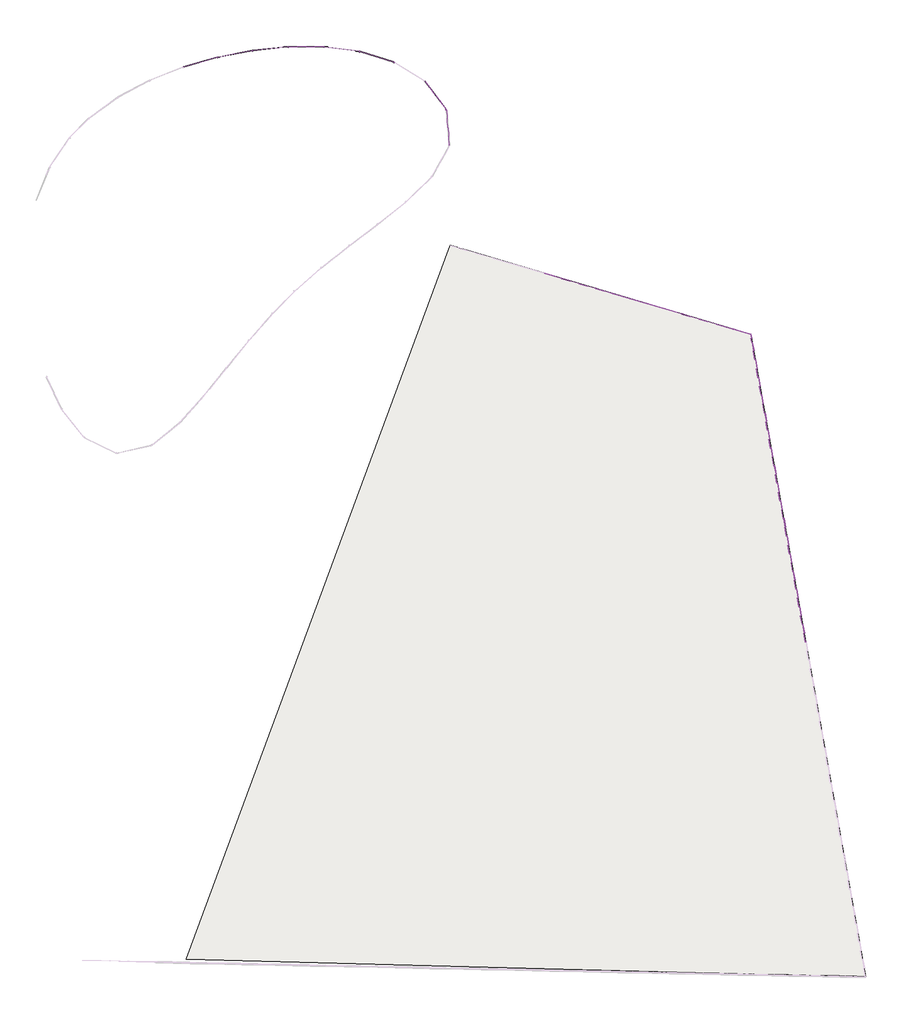
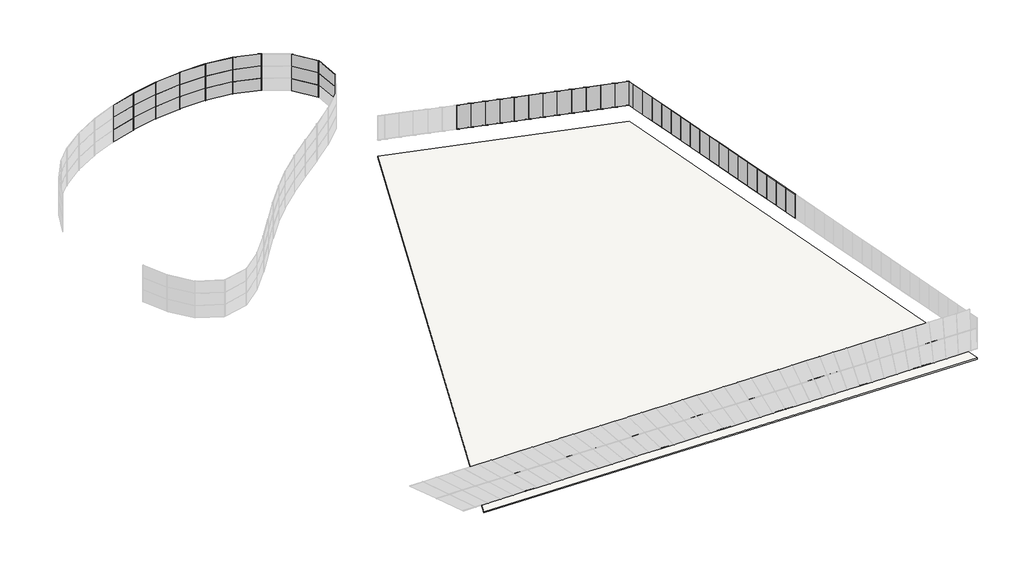
# One storey, part 5 of 5: 53 plates, 51 members, 1 slab.
"""IFC4 building model written with IfcOpenShell, lengths in millimetres."""

import ifcopenshell
import ifcopenshell.guid

model = None  # the IFC model being written
_history = None  # IfcOwnerHistory: only IFC2X3 demands one
_inside = {}  # id of a spatial element -> (the spatial element, [elements in it])
_under = {}  # id of a project, library or spatial element -> (it, [spatial elements below it])
_declared = {}  # id of a project -> (the project, [libraries it declares])
_typed = {}  # id of a type object -> (the type object, [elements of that type])
_made_of = {}  # id of a material, layer set ... -> (it, [elements and type objects made of it])


def new_model(schema):
    """Start an empty IFC model of exactly this schema.

    Asked for "IFC4X3", IfcOpenShell would pick the latest addendum, in which some entities
    have other attributes; the version numbers below select the first issue.
    IFC2X3 requires an IfcOwnerHistory on every rooted entity: one is made here for all.
    """
    global model, _history
    if schema == "IFC4X3":
        model = ifcopenshell.file(schema_version=(4, 3, 0, 0))
    else:
        model = ifcopenshell.file(schema=schema)
    _inside.clear()
    _under.clear()
    _declared.clear()
    _typed.clear()
    _made_of.clear()
    _history = None
    if model.schema == "IFC2X3":
        org = make("IfcOrganization", Name="unknown")
        user = make(
            "IfcPersonAndOrganization",
            ThePerson=make("IfcPerson", FamilyName="unknown"),
            TheOrganization=org,
        )
        app = make(
            "IfcApplication",
            ApplicationDeveloper=org,
            Version="unknown",
            ApplicationFullName="unknown",
            ApplicationIdentifier="unknown",
        )
        _history = make(
            "IfcOwnerHistory",
            OwningUser=user,
            OwningApplication=app,
            ChangeAction="ADDED",
            CreationDate=0,
        )
    return model


def make(cls, **values):
    """One entity of the class cls with the attributes given. An attribute that is None is left unset."""
    return model.create_entity(
        cls, **{name: value for name, value in values.items() if value is not None}
    )


def rooted(cls, **values):
    """An entity with a GlobalId (a new one), such as an element, a storey or a relation."""
    return make(cls, GlobalId=ifcopenshell.guid.new(), OwnerHistory=_history, **values)


def si_unit(unit_type, name, prefix=None):
    """IfcSIUnit, for example si_unit("LENGTHUNIT", "METRE", prefix="MILLI")."""
    return make("IfcSIUnit", UnitType=unit_type, Prefix=prefix, Name=name)


def assignment(units):
    """IfcUnitAssignment: the units of a project."""
    return None if units is None else make("IfcUnitAssignment", Units=units)


def point(xyz):
    """IfcCartesianPoint."""
    return None if xyz is None else make("IfcCartesianPoint", Coordinates=xyz)


def direction(xyz):
    """IfcDirection."""
    return None if xyz is None else make("IfcDirection", DirectionRatios=xyz)


def frame(location, z_axis=None, x_axis=None):
    """IfcAxis2Placement3D, a coordinate frame: its origin and axes. An axis left out is left unset."""
    return make(
        "IfcAxis2Placement3D",
        Location=point(location),
        Axis=direction(z_axis),
        RefDirection=direction(x_axis),
    )


def frame_2d(location, x_axis=None):
    """IfcAxis2Placement2D, a coordinate frame in the plane: its origin and x axis."""
    return make(
        "IfcAxis2Placement2D", Location=point(location), RefDirection=direction(x_axis)
    )


def origin():
    """The frame at (0, 0, 0) with its axes left unset."""
    return frame((0.0, 0.0, 0.0))


def origin_with_axes():
    """The frame at (0, 0, 0) with the z axis (0, 0, 1) and the x axis (1, 0, 0) written out."""
    return frame((0.0, 0.0, 0.0), z_axis=(0.0, 0.0, 1.0), x_axis=(1.0, 0.0, 0.0))


def origin_2d():
    """The frame at (0, 0) in the plane with its x axis left unset."""
    return frame_2d((0.0, 0.0))


def place(relative_to, where):
    """IfcLocalPlacement: puts the frame where relative to a parent placement (None: the world)."""
    return make(
        "IfcLocalPlacement", PlacementRelTo=relative_to, RelativePlacement=where
    )


def context(
    kind, dimensions, precision=None, world=None, true_north=None, identifier=None
):
    """IfcGeometricRepresentationContext, for example the 3D "Model" context."""
    return make(
        "IfcGeometricRepresentationContext",
        ContextIdentifier=identifier,
        ContextType=kind,
        CoordinateSpaceDimension=dimensions,
        Precision=precision,
        WorldCoordinateSystem=world,
        TrueNorth=true_north,
    )


def project(units=None, contexts=None):
    """IfcProject with its units and contexts."""
    return rooted(
        "IfcProject",
        Name="project",
        RepresentationContexts=contexts,
        UnitsInContext=assignment(units),
    )


def spatial(cls, under=None, at=None, **own):
    """A site, building, storey or space (cls), placed at a placement, below another one or the project."""
    s = rooted(cls, ObjectPlacement=at, **own)
    if under is not None:
        _under.setdefault(under.id(), (under, []))[1].append(s)
    return s


def polyline(points):
    """IfcPolyline through the points."""
    return make("IfcPolyline", Points=[point(p) for p in points])


def circle_curve(where, radius):
    """IfcCircle in the frame where."""
    return make("IfcCircle", Position=where, Radius=radius)


def trimmed(basis, trim1, trim2, sense, master):
    """IfcTrimmedCurve: the piece of a basis curve between two trims."""
    return make(
        "IfcTrimmedCurve",
        BasisCurve=basis,
        Trim1=trim1,
        Trim2=trim2,
        SenseAgreement=sense,
        MasterRepresentation=master,
    )


def segment(curve, same_sense, transition):
    """IfcCompositeCurveSegment."""
    return make(
        "IfcCompositeCurveSegment",
        Transition=transition,
        SameSense=same_sense,
        ParentCurve=curve,
    )


def composite_curve(segments, self_intersect=None):
    """IfcCompositeCurve: segments joined end to end."""
    return make("IfcCompositeCurve", Segments=segments, SelfIntersect=self_intersect)


def outline(outer, holes=None, kind="AREA"):
    """IfcArbitraryClosedProfileDef: a profile drawn as a closed curve; with holes, ...WithVoids."""
    if holes is None:
        return make("IfcArbitraryClosedProfileDef", ProfileType=kind, OuterCurve=outer)
    return make(
        "IfcArbitraryProfileDefWithVoids",
        ProfileType=kind,
        OuterCurve=outer,
        InnerCurves=holes,
    )


def extrude(swept, where, along, depth):
    """IfcExtrudedAreaSolid: the profile swept, set in the frame where, extruded along a direction by depth."""
    return make(
        "IfcExtrudedAreaSolid",
        SweptArea=swept,
        Position=where,
        ExtrudedDirection=direction(along),
        Depth=depth,
    )


def shape(context_of_items, identifier, shape_type, items):
    """IfcShapeRepresentation: the items that make up one representation, for example the "Body"."""
    return make(
        "IfcShapeRepresentation",
        ContextOfItems=context_of_items,
        RepresentationIdentifier=identifier,
        RepresentationType=shape_type,
        Items=items,
    )


def source(mapping_origin, context_of_items, identifier, shape_type, items):
    """IfcRepresentationMap: a shape defined once, which mapped items show again and again."""
    return make(
        "IfcRepresentationMap",
        MappingOrigin=mapping_origin,
        MappedRepresentation=shape(context_of_items, identifier, shape_type, items),
    )


def transform(
    local_origin,
    x_axis=None,
    y_axis=None,
    z_axis=None,
    scale=None,
    scale2=None,
    scale3=None,
    uniform=True,
):
    """IfcCartesianTransformationOperator3D, or its non-uniform kind. x_axis, y_axis, z_axis: its Axis1, 2, 3."""
    if uniform:
        return make(
            "IfcCartesianTransformationOperator3D",
            Axis1=direction(x_axis),
            Axis2=direction(y_axis),
            LocalOrigin=point(local_origin),
            Scale=scale,
            Axis3=direction(z_axis),
        )
    return make(
        "IfcCartesianTransformationOperator3DnonUniform",
        Axis1=direction(x_axis),
        Axis2=direction(y_axis),
        LocalOrigin=point(local_origin),
        Scale=scale,
        Axis3=direction(z_axis),
        Scale2=scale2,
        Scale3=scale3,
    )


def mapped(mapping_source, mapping_target):
    """IfcMappedItem: shows the shape of a source again, moved by a transform."""
    return make(
        "IfcMappedItem", MappingSource=mapping_source, MappingTarget=mapping_target
    )


def made_of(thing, what):
    """Note that an element or type object is made of a material, layer set ...; save() writes the relation."""
    if what is not None:
        _made_of.setdefault(what.id(), (what, []))[1].append(thing)
    return thing


def element(
    cls,
    number,
    at=None,
    inside=None,
    cuts=None,
    type_object=None,
    material=None,
    context=None,
    identifier="Body",
    shape_type=None,
    held_by="IfcProductDefinitionShape",
    body=None,
    shapes=None,
    **own,
):
    """One element of the class cls, such as IfcWall. Its Tag is "e" and its number.

    at: its placement. inside: the storey or other place that contains it. cuts: it is an
    opening in that element (IfcRelVoidsElement). A single representation is given by context,
    identifier, shape_type and body (its items); several are given by shapes. held_by: the class
    of the entity that holds the representations. save() writes the other relations.
    """
    e = rooted(cls, Tag="e%d" % number, ObjectPlacement=at, **own)
    if body is not None:
        shapes = [shape(context, identifier, shape_type, body)]
    if shapes is not None:
        e.Representation = make(held_by, Representations=shapes)
    if inside is not None:
        _inside.setdefault(inside.id(), (inside, []))[1].append(e)
    if cuts is not None:
        rooted(
            "IfcRelVoidsElement", RelatingBuildingElement=cuts, RelatedOpeningElement=e
        )
    if type_object is not None:
        _typed.setdefault(type_object.id(), (type_object, []))[1].append(e)
    return made_of(e, material)


def aggregate(whole, parts):
    """IfcRelAggregates: a whole, such as a stair, and the parts it consists of."""
    return rooted("IfcRelAggregates", RelatingObject=whole, RelatedObjects=parts)


def save(model, path):
    """Write the relations noted so far, then the file.

    IfcRelAggregates (storeys below a building ...), IfcRelContainedInSpatialStructure (elements
    in a storey), IfcRelDefinesByType, IfcRelAssociatesMaterial and IfcRelDeclares: one each for
    every whole, place, type object, material and project.
    """
    for whole, parts in _under.values():
        aggregate(whole, parts)
    for where, things in _inside.values():
        rooted(
            "IfcRelContainedInSpatialStructure",
            RelatedElements=things,
            RelatingStructure=where,
        )
    for kind, things in _typed.values():
        rooted("IfcRelDefinesByType", RelatedObjects=things, RelatingType=kind)
    for what, things in _made_of.values():
        rooted("IfcRelAssociatesMaterial", RelatedObjects=things, RelatingMaterial=what)
    for by, libraries in _declared.values():
        rooted("IfcRelDeclares", RelatingContext=by, RelatedDefinitions=libraries)
    model.write(path)


def montante_circular_25_mm_raio_36e581cf(model_context):
    return source(origin(), model_context, "Body", "SweptSolid", [
        extrude(outline(composite_curve([segment(trimmed(circle_curve(origin_2d(), 25.0), [point((25.0, 0.0))], [point((-25.0, 0.0))], False, "CARTESIAN"), True, "CONTINUOUS"), segment(trimmed(circle_curve(origin_2d(), 25.0), [point((-25.0, 0.0))], [point((25.0, 0.0))], False, "CARTESIAN"), True, "CONTINUOUS")], self_intersect=False)), frame((0.0, 0.0, -1500.0), z_axis=(0.0, 0.0, 1.0), x_axis=(1.0, 0.0, 0.0)), (0.0, 0.0, 1.0), 1500.0),
    ])


def montante_circular_25_mm_raio_b6a72e74(model_context):
    return source(origin(), model_context, "Body", "SweptSolid", [
        extrude(outline(composite_curve([segment(trimmed(circle_curve(origin_2d(), 25.0), [point((25.0, 0.0))], [point((-25.0, 0.0))], False, "CARTESIAN"), True, "CONTINUOUS"), segment(trimmed(circle_curve(origin_2d(), 25.0), [point((-25.0, 0.0))], [point((25.0, 0.0))], False, "CARTESIAN"), True, "CONTINUOUS")], self_intersect=False)), frame((0.0, 0.0, -685.7133319), z_axis=(0.0, 0.0, 1.0), x_axis=(1.0, 0.0, 0.0)), (0.0, 0.0, 1.0), 685.7133319),
    ])


def painel_do_sistema_5ef9eced(model_context):
    return source(origin(), model_context, "Body", "SweptSolid", [
        extrude(outline(polyline([(1475.0, 24.5), (-1475.0, 24.5), (-1475.0, 49.5), (1475.0, 49.5), (1475.0, 24.5)])), origin_with_axes(), (0.0, 0.0, 1.0), 1500.0),
    ])


def painel_do_sistema_14e00207(model_context):
    return source(origin(), model_context, "Body", "SweptSolid", [
        extrude(outline(polyline([(1475.0, 24.5), (-1475.0, 24.5), (-1475.0, 49.5), (1475.0, 49.5), (1475.0, 24.5)])), origin_with_axes(), (0.0, 0.0, 1.0), 685.7133319),
    ])


def painel_do_sistema_85ccde5d(model_context):
    return source(origin(), model_context, "Body", "SweptSolid", [
        extrude(outline(polyline([(1475.0, -49.5), (-1475.0, -49.5), (-1475.0, -24.5), (1475.0, -24.5), (1475.0, -49.5)])), origin_with_axes(), (0.0, 0.0, 1.0), 1500.0),
    ])


model = new_model("IFC4")

# Units and contexts
model_context = context("Model", 3, world=origin())
ifc_project = project(units=[si_unit("LENGTHUNIT", "METRE", prefix="MILLI")], contexts=[model_context])

# Site, building, storey
site = spatial("IfcSite", under=ifc_project)
building = spatial("IfcBuilding", under=site)
storey = spatial("IfcBuildingStorey", under=building, Name="Nível 2", Elevation=4000.0)

# Members
placement = place(None, origin())
montante_circular_25_mm_raio_shape = montante_circular_25_mm_raio_36e581cf(model_context)
element("IfcMember", 1, ObjectType="Montante circular : 25 mm Raio", at=placement, inside=storey, context=model_context, shape_type="MappedRepresentation", body=[
    mapped(montante_circular_25_mm_raio_shape, transform((17189.2092362, 25994.5128335, 6000.000015), x_axis=(0.0, 0.0, 1.0), y_axis=(0.2831837893953463, 0.9590656606425298, 0.0), z_axis=(-0.9590656606425297, 0.2831837893953462, 0.0))),
])
element("IfcMember", 2, ObjectType="Montante circular : 25 mm Raio", at=placement, inside=storey, context=model_context, shape_type="MappedRepresentation", body=[
    mapped(montante_circular_25_mm_raio_shape, transform((22977.759166, 1270.3057737, 6000.000015), x_axis=(0.0, 0.0, 1.0), y_axis=(0.9843520034862604, 0.17621331740985194, 0.0), z_axis=(-0.17621331740985194, 0.9843520034862604, 0.0))),
])
element("IfcMember", 3, ObjectType="Montante circular : 25 mm Raio", at=placement, inside=storey, context=model_context, shape_type="MappedRepresentation", body=[
    mapped(montante_circular_25_mm_raio_shape, transform((22713.4391899, 2746.833779, 6000.000015), x_axis=(0.0, 0.0, 1.0), y_axis=(0.9843520034862615, 0.17621331740984614, 0.0), z_axis=(-0.1762133174098461, 0.9843520034862614, 0.0))),
])
element("IfcMember", 4, ObjectType="Montante circular : 25 mm Raio", at=placement, inside=storey, context=model_context, shape_type="MappedRepresentation", body=[
    mapped(montante_circular_25_mm_raio_shape, transform((22449.1192138, 4223.3617842, 6000.000015), x_axis=(0.0, 0.0, 1.0), y_axis=(0.9843520034862611, 0.17621331740984805, 0.0), z_axis=(-0.17621331740984805, 0.9843520034862611, 0.0))),
])
element("IfcMember", 5, ObjectType="Montante circular : 25 mm Raio", at=placement, inside=storey, context=model_context, shape_type="MappedRepresentation", body=[
    mapped(montante_circular_25_mm_raio_shape, transform((22184.7992376, 5699.8897894, 6000.000015), x_axis=(0.0, 0.0, 1.0), y_axis=(0.9843520034862614, 0.17621331740984636, 0.0), z_axis=(-0.17621331740984636, 0.9843520034862614, 0.0))),
])
element("IfcMember", 6, ObjectType="Montante circular : 25 mm Raio", at=placement, inside=storey, context=model_context, shape_type="MappedRepresentation", body=[
    mapped(montante_circular_25_mm_raio_shape, transform((21920.4792615, 7176.4177946, 6000.000015), x_axis=(0.0, 0.0, 1.0), y_axis=(0.9843520034862608, 0.17621331740984977, 0.0), z_axis=(-0.17621331740984977, 0.9843520034862608, 0.0))),
])
element("IfcMember", 7, ObjectType="Montante circular : 25 mm Raio", at=placement, inside=storey, context=model_context, shape_type="MappedRepresentation", body=[
    mapped(montante_circular_25_mm_raio_shape, transform((21656.1592854, 8652.9457999, 6000.000015), x_axis=(0.0, 0.0, 1.0), y_axis=(0.9843520034862612, 0.17621331740984747, 0.0), z_axis=(-0.17621331740984747, 0.9843520034862612, 0.0))),
])
element("IfcMember", 8, ObjectType="Montante circular : 25 mm Raio", at=placement, inside=storey, context=model_context, shape_type="MappedRepresentation", body=[
    mapped(montante_circular_25_mm_raio_shape, transform((21391.8393093, 10129.4738051, 6000.000015), x_axis=(0.0, 0.0, 1.0), y_axis=(0.9843520034862608, 0.17621331740984966, 0.0), z_axis=(-0.17621331740984966, 0.9843520034862608, 0.0))),
])
element("IfcMember", 9, ObjectType="Montante circular : 25 mm Raio", at=placement, inside=storey, context=model_context, shape_type="MappedRepresentation", body=[
    mapped(montante_circular_25_mm_raio_shape, transform((21127.5193332, 11606.0018103, 6000.000015), x_axis=(0.0, 0.0, 1.0), y_axis=(0.9843520034862614, 0.17621331740984636, 0.0), z_axis=(-0.17621331740984636, 0.9843520034862614, 0.0))),
])
element("IfcMember", 10, ObjectType="Montante circular : 25 mm Raio", at=placement, inside=storey, context=model_context, shape_type="MappedRepresentation", body=[
    mapped(montante_circular_25_mm_raio_shape, transform((20863.1993571, 13082.5298156, 6000.000015), x_axis=(0.0, 0.0, 1.0), y_axis=(0.9843520034862611, 0.17621331740984836, 0.0), z_axis=(-0.17621331740984836, 0.9843520034862611, 0.0))),
])
element("IfcMember", 11, ObjectType="Montante circular : 25 mm Raio", at=placement, inside=storey, context=model_context, shape_type="MappedRepresentation", body=[
    mapped(montante_circular_25_mm_raio_shape, transform((20598.8793809, 14559.0578208, 6000.000015), x_axis=(0.0, 0.0, 1.0), y_axis=(0.9843520034862613, 0.17621331740984736, 0.0), z_axis=(-0.17621331740984733, 0.9843520034862612, 0.0))),
])
element("IfcMember", 12, ObjectType="Montante circular : 25 mm Raio", at=placement, inside=storey, context=model_context, shape_type="MappedRepresentation", body=[
    mapped(montante_circular_25_mm_raio_shape, transform((20334.5594048, 16035.585826, 6000.000015), x_axis=(0.0, 0.0, 1.0), y_axis=(0.9843520034862608, 0.17621331740984966, 0.0), z_axis=(-0.17621331740984966, 0.9843520034862608, 0.0))),
])
element("IfcMember", 13, ObjectType="Montante circular : 25 mm Raio", at=placement, inside=storey, context=model_context, shape_type="MappedRepresentation", body=[
    mapped(montante_circular_25_mm_raio_shape, transform((20070.2394287, 17512.1138312, 6000.000015), x_axis=(0.0, 0.0, 1.0), y_axis=(0.9843520034862613, 0.1762133174098471, 0.0), z_axis=(-0.17621331740984708, 0.9843520034862612, 0.0))),
])
element("IfcMember", 14, ObjectType="Montante circular : 25 mm Raio", at=placement, inside=storey, context=model_context, shape_type="MappedRepresentation", body=[
    mapped(montante_circular_25_mm_raio_shape, transform((19805.9194526, 18988.6418365, 6000.000015), x_axis=(0.0, 0.0, 1.0), y_axis=(0.9843520034862611, 0.17621331740984836, 0.0), z_axis=(-0.17621331740984836, 0.9843520034862611, 0.0))),
])
element("IfcMember", 15, ObjectType="Montante circular : 25 mm Raio", at=placement, inside=storey, context=model_context, shape_type="MappedRepresentation", body=[
    mapped(montante_circular_25_mm_raio_shape, transform((19541.5994765, 20465.1698417, 6000.000015), x_axis=(0.0, 0.0, 1.0), y_axis=(0.9843520034862608, 0.1762133174098494, 0.0), z_axis=(-0.1762133174098494, 0.9843520034862608, 0.0))),
])
element("IfcMember", 16, ObjectType="Montante circular : 25 mm Raio", at=placement, inside=storey, context=model_context, shape_type="MappedRepresentation", body=[
    mapped(montante_circular_25_mm_raio_shape, transform((19277.2795004, 21941.6978469, 6000.000015), x_axis=(0.0, 0.0, 1.0), y_axis=(0.9843520034862612, 0.1762133174098476, 0.0), z_axis=(-0.1762133174098476, 0.9843520034862612, 0.0))),
])
element("IfcMember", 17, ObjectType="Montante circular : 25 mm Raio", at=placement, inside=storey, context=model_context, shape_type="MappedRepresentation", body=[
    mapped(montante_circular_25_mm_raio_shape, transform((19012.9595243, 23418.2258522, 6000.000015), x_axis=(0.0, 0.0, 1.0), y_axis=(0.9843520034862611, 0.1762133174098481, 0.0), z_axis=(-0.1762133174098481, 0.9843520034862611, 0.0))),
])
element("IfcMember", 18, ObjectType="Montante circular : 25 mm Raio", at=placement, inside=storey, context=model_context, shape_type="MappedRepresentation", body=[
    mapped(montante_circular_25_mm_raio_shape, transform((18748.6395481, 24894.7538574, 6000.000015), x_axis=(0.0, 0.0, 1.0), y_axis=(0.9843520034862611, 0.1762133174098484, 0.0), z_axis=(-0.17621331740984839, 0.984352003486261, 0.0))),
])
element("IfcMember", 19, ObjectType="Montante circular : 25 mm Raio", at=placement, inside=storey, context=model_context, shape_type="MappedRepresentation", body=[
    mapped(montante_circular_25_mm_raio_shape, transform((15750.6107452, 26419.2885176, 6000.000015), x_axis=(0.0, 0.0, 1.0), y_axis=(0.28318378939534644, 0.9590656606425298, 0.0), z_axis=(-0.9590656606425298, 0.28318378939534644, 0.0))),
])
element("IfcMember", 20, ObjectType="Montante circular : 25 mm Raio", at=placement, inside=storey, context=model_context, shape_type="MappedRepresentation", body=[
    mapped(montante_circular_25_mm_raio_shape, transform((14312.0122543, 26844.0642017, 6000.000015), x_axis=(0.0, 0.0, 1.0), y_axis=(0.2831837893953491, 0.959065660642529, 0.0), z_axis=(-0.959065660642529, 0.2831837893953491, 0.0))),
])
element("IfcMember", 21, ObjectType="Montante circular : 25 mm Raio", at=placement, inside=storey, context=model_context, shape_type="MappedRepresentation", body=[
    mapped(montante_circular_25_mm_raio_shape, transform((12873.4137633, 27268.8398858, 6000.000015), x_axis=(0.0, 0.0, 1.0), y_axis=(0.2831837893953487, 0.9590656606425292, 0.0), z_axis=(-0.9590656606425291, 0.28318378939534866, 0.0))),
])
element("IfcMember", 22, ObjectType="Montante circular : 25 mm Raio", at=placement, inside=storey, context=model_context, shape_type="MappedRepresentation", body=[
    mapped(montante_circular_25_mm_raio_shape, transform((11434.8152723, 27693.6155699, 6000.000015), x_axis=(0.0, 0.0, 1.0), y_axis=(0.2831837893953472, 0.9590656606425295, 0.0), z_axis=(-0.9590656606425295, 0.2831837893953472, 0.0))),
])
element("IfcMember", 23, ObjectType="Montante circular : 25 mm Raio", at=placement, inside=storey, context=model_context, shape_type="MappedRepresentation", body=[
    mapped(montante_circular_25_mm_raio_shape, transform((9996.2167814, 28118.391254, 6000.000015), x_axis=(0.0, 0.0, 1.0), y_axis=(0.2831837893953487, 0.9590656606425292, 0.0), z_axis=(-0.9590656606425291, 0.28318378939534866, 0.0))),
])
element("IfcMember", 24, ObjectType="Montante circular : 25 mm Raio", at=placement, inside=storey, context=model_context, shape_type="MappedRepresentation", body=[
    mapped(montante_circular_25_mm_raio_shape, transform((8557.6182904, 28543.1669381, 6000.000015), x_axis=(0.0, 0.0, 1.0), y_axis=(0.28318378939534666, 0.9590656606425297, 0.0), z_axis=(-0.9590656606425296, 0.2831837893953466, 0.0))),
])
element("IfcMember", 25, ObjectType="Montante circular : 25 mm Raio", at=placement, inside=storey, context=model_context, shape_type="MappedRepresentation", body=[
    mapped(montante_circular_25_mm_raio_shape, transform((7119.0197994, 28967.9426222, 6000.000015), x_axis=(0.0, 0.0, 1.0), y_axis=(0.2831837893953493, 0.959065660642529, 0.0), z_axis=(-0.959065660642529, 0.2831837893953493, 0.0))),
])
element("IfcMember", 26, ObjectType="Montante circular : 25 mm Raio", at=placement, inside=storey, context=model_context, shape_type="MappedRepresentation", body=[
    mapped(montante_circular_25_mm_raio_shape, transform((5680.4213085, 29392.7183063, 6000.000015), x_axis=(0.0, 0.0, 1.0), y_axis=(0.2831837893953491, 0.959065660642529, 0.0), z_axis=(-0.959065660642529, 0.2831837893953491, 0.0))),
])
element("IfcMember", 27, ObjectType="Montante circular : 25 mm Raio", at=placement, inside=storey, context=model_context, shape_type="MappedRepresentation", body=[
    mapped(montante_circular_25_mm_raio_shape, transform((4241.8228175, 29817.4939904, 6000.000015), x_axis=(0.0, 0.0, 1.0), y_axis=(0.28318378939534394, 0.9590656606425305, 0.0), z_axis=(-0.9590656606425305, 0.28318378939534394, 0.0))),
])
element("IfcMember", 28, ObjectType="Montante circular : 25 mm Raio", at=placement, inside=storey, context=model_context, shape_type="MappedRepresentation", body=[
    mapped(montante_circular_25_mm_raio_shape, transform((2803.2243265, 30242.2696745, 6000.000015), x_axis=(0.0, 0.0, 1.0), y_axis=(0.28318378939535055, 0.9590656606425285, 0.0), z_axis=(-0.9590656606425285, 0.28318378939535055, 0.0))),
])
element("IfcMember", 29, ObjectType="Montante circular : 25 mm Raio", at=placement, inside=storey, context=model_context, shape_type="MappedRepresentation", body=[
    mapped(montante_circular_25_mm_raio_shape, transform((1364.6258356, 30667.0453586, 6000.000015), x_axis=(0.0, 0.0, 1.0), y_axis=(0.28318378939534644, 0.9590656606425298, 0.0), z_axis=(-0.9590656606425298, 0.28318378939534644, 0.0))),
])
element("IfcMember", 30, ObjectType="Montante circular : 25 mm Raio", at=placement, inside=storey, context=model_context, shape_type="MappedRepresentation", body=[
    mapped(montante_circular_25_mm_raio_shape, transform((-6868.5829053, 44343.271676, 4500.0), x_axis=(-0.3894872634933398, 0.9210318515537178, 0.0), y_axis=(0.9210318515537178, 0.3894872634933398, 0.0), z_axis=(0.0, 0.0, -1.0))),
])
element("IfcMember", 31, ObjectType="Montante circular : 25 mm Raio", at=placement, inside=storey, context=model_context, shape_type="MappedRepresentation", body=[
    mapped(montante_circular_25_mm_raio_shape, transform((-11244.034472, 48297.0103794, 4500.0), x_axis=(-0.9160451113541028, 0.40107524725947563, 0.0), y_axis=(0.40107524725947563, 0.9160451113541028, 0.0), z_axis=(0.0, 0.0, -1.0))),
])
element("IfcMember", 32, ObjectType="Montante circular : 25 mm Raio", at=placement, inside=storey, context=model_context, shape_type="MappedRepresentation", body=[
    mapped(montante_circular_25_mm_raio_shape, transform((-14105.1754803, 49199.1589981, 4500.0), x_axis=(-0.9782677823869713, 0.20734547485700608, 0.0), y_axis=(0.20734547485700608, 0.9782677823869713, 0.0), z_axis=(0.0, 0.0, -1.0))),
])
element("IfcMember", 33, ObjectType="Montante circular : 25 mm Raio", at=placement, inside=storey, context=model_context, shape_type="MappedRepresentation", body=[
    mapped(montante_circular_25_mm_raio_shape, transform((-17080.2416106, 49585.140242, 4500.0), x_axis=(-0.998380379517221, 0.0568912804834772, 0.0), y_axis=(0.0568912804834772, 0.998380379517221, 0.0), z_axis=(0.0, 0.0, -1.0))),
])
element("IfcMember", 34, ObjectType="Montante circular : 25 mm Raio", at=placement, inside=storey, context=model_context, shape_type="MappedRepresentation", body=[
    mapped(montante_circular_25_mm_raio_shape, transform((-20080.239517, 49581.5960042, 4500.0), x_axis=(-0.9985092878419478, -0.054582067507252724, 0.0), y_axis=(-0.054582067507252724, 0.9985092878419478, 0.0), z_axis=(0.0, 0.0, -1.0))),
])
element("IfcMember", 35, ObjectType="Montante circular : 25 mm Raio", at=placement, inside=storey, context=model_context, shape_type="MappedRepresentation", body=[
    mapped(montante_circular_25_mm_raio_shape, transform((-23064.637889, 49276.0369149, 4500.0), x_axis=(-0.9891120775870231, -0.14716418712269272, 0.0), y_axis=(-0.14716418712269272, 0.9891120775870231, 0.0), z_axis=(0.0, 0.0, -1.0))),
])
element("IfcMember", 36, ObjectType="Montante circular : 25 mm Raio", at=placement, inside=storey, context=model_context, shape_type="MappedRepresentation", body=[
    mapped(montante_circular_25_mm_raio_shape, transform((-26009.7169515, 48704.6269783, 4500.0), x_axis=(-0.9724041864044524, -0.23330258949076224, 0.0), y_axis=(-0.23330258949076224, 0.9724041864044524, 0.0), z_axis=(0.0, 0.0, -1.0))),
])
element("IfcMember", 37, ObjectType="Montante circular : 25 mm Raio", at=placement, inside=storey, context=model_context, shape_type="MappedRepresentation", body=[
    mapped(montante_circular_25_mm_raio_shape, transform((-6868.5829053, 44343.271676, 6000.0), x_axis=(-0.38948726349333984, 0.9210318515537178, 0.0), y_axis=(0.9210318515537178, 0.38948726349333984, 0.0), z_axis=(0.0, 0.0, -1.0))),
])
element("IfcMember", 38, ObjectType="Montante circular : 25 mm Raio", at=placement, inside=storey, context=model_context, shape_type="MappedRepresentation", body=[
    mapped(montante_circular_25_mm_raio_shape, transform((-11244.034472, 48297.0103794, 6000.0), x_axis=(-0.9160451113541028, 0.40107524725947563, 0.0), y_axis=(0.40107524725947563, 0.9160451113541028, 0.0), z_axis=(0.0, 0.0, -1.0))),
])
element("IfcMember", 39, ObjectType="Montante circular : 25 mm Raio", at=placement, inside=storey, context=model_context, shape_type="MappedRepresentation", body=[
    mapped(montante_circular_25_mm_raio_shape, transform((-14105.1754803, 49199.1589981, 6000.0), x_axis=(-0.9782677823869713, 0.20734547485700608, 0.0), y_axis=(0.20734547485700608, 0.9782677823869713, 0.0), z_axis=(0.0, 0.0, -1.0))),
])
element("IfcMember", 40, ObjectType="Montante circular : 25 mm Raio", at=placement, inside=storey, context=model_context, shape_type="MappedRepresentation", body=[
    mapped(montante_circular_25_mm_raio_shape, transform((-17080.2416106, 49585.140242, 6000.0), x_axis=(-0.998380379517221, 0.0568912804834772, 0.0), y_axis=(0.0568912804834772, 0.998380379517221, 0.0), z_axis=(0.0, 0.0, -1.0))),
])
element("IfcMember", 41, ObjectType="Montante circular : 25 mm Raio", at=placement, inside=storey, context=model_context, shape_type="MappedRepresentation", body=[
    mapped(montante_circular_25_mm_raio_shape, transform((-20080.239517, 49581.5960042, 6000.0), x_axis=(-0.9985092878419478, -0.05458206750725284, 0.0), y_axis=(-0.05458206750725284, 0.9985092878419478, 0.0), z_axis=(0.0, 0.0, -1.0))),
])
element("IfcMember", 42, ObjectType="Montante circular : 25 mm Raio", at=placement, inside=storey, context=model_context, shape_type="MappedRepresentation", body=[
    mapped(montante_circular_25_mm_raio_shape, transform((-23064.637889, 49276.0369149, 6000.0), x_axis=(-0.989112077587023, -0.14716418712269302, 0.0), y_axis=(-0.14716418712269302, 0.989112077587023, 0.0), z_axis=(0.0, 0.0, -1.0))),
])
element("IfcMember", 43, ObjectType="Montante circular : 25 mm Raio", at=placement, inside=storey, context=model_context, shape_type="MappedRepresentation", body=[
    mapped(montante_circular_25_mm_raio_shape, transform((-26009.7169515, 48704.6269783, 6000.0), x_axis=(-0.9724041864044525, -0.2333025894907617, 0.0), y_axis=(-0.2333025894907617, 0.9724041864044525, 0.0), z_axis=(0.0, 0.0, -1.0))),
])
element("IfcMember", 44, ObjectType="Montante circular : 25 mm Raio", at=placement, inside=storey, context=model_context, shape_type="MappedRepresentation", body=[
    mapped(montante_circular_25_mm_raio_shape, transform((-6868.5829053, 44343.271676, 7500.0), x_axis=(-0.3894872634933398, 0.9210318515537178, 0.0), y_axis=(0.9210318515537178, 0.3894872634933398, 0.0), z_axis=(0.0, 0.0, -1.0))),
])
element("IfcMember", 45, ObjectType="Montante circular : 25 mm Raio", at=placement, inside=storey, context=model_context, shape_type="MappedRepresentation", body=[
    mapped(montante_circular_25_mm_raio_shape, transform((-11244.034472, 48297.0103794, 7500.0), x_axis=(-0.9160451113541028, 0.40107524725947563, 0.0), y_axis=(0.40107524725947563, 0.9160451113541028, 0.0), z_axis=(0.0, 0.0, -1.0))),
])
element("IfcMember", 46, ObjectType="Montante circular : 25 mm Raio", at=placement, inside=storey, context=model_context, shape_type="MappedRepresentation", body=[
    mapped(montante_circular_25_mm_raio_shape, transform((-14105.1754803, 49199.1589981, 7500.0), x_axis=(-0.9782677823869713, 0.20734547485700608, 0.0), y_axis=(0.20734547485700608, 0.9782677823869713, 0.0), z_axis=(0.0, 0.0, -1.0))),
])
element("IfcMember", 47, ObjectType="Montante circular : 25 mm Raio", at=placement, inside=storey, context=model_context, shape_type="MappedRepresentation", body=[
    mapped(montante_circular_25_mm_raio_shape, transform((-17080.2416106, 49585.140242, 7500.0), x_axis=(-0.998380379517221, 0.0568912804834772, 0.0), y_axis=(0.0568912804834772, 0.998380379517221, 0.0), z_axis=(0.0, 0.0, -1.0))),
])
element("IfcMember", 48, ObjectType="Montante circular : 25 mm Raio", at=placement, inside=storey, context=model_context, shape_type="MappedRepresentation", body=[
    mapped(montante_circular_25_mm_raio_shape, transform((-20080.239517, 49581.5960042, 7500.0), x_axis=(-0.9985092878419478, -0.054582067507252724, 0.0), y_axis=(-0.054582067507252724, 0.9985092878419478, 0.0), z_axis=(0.0, 0.0, -1.0))),
])
element("IfcMember", 49, ObjectType="Montante circular : 25 mm Raio", at=placement, inside=storey, context=model_context, shape_type="MappedRepresentation", body=[
    mapped(montante_circular_25_mm_raio_shape, transform((-23064.637889, 49276.0369149, 7500.0), x_axis=(-0.989112077587023, -0.14716418712269305, 0.0), y_axis=(-0.14716418712269305, 0.989112077587023, 0.0), z_axis=(0.0, 0.0, -1.0))),
])
element("IfcMember", 50, ObjectType="Montante circular : 25 mm Raio", at=placement, inside=storey, context=model_context, shape_type="MappedRepresentation", body=[
    mapped(montante_circular_25_mm_raio_shape, transform((-26009.7169515, 48704.6269783, 7500.0), x_axis=(-0.9724041864044524, -0.23330258949076224, 0.0), y_axis=(-0.23330258949076224, 0.9724041864044524, 0.0), z_axis=(0.0, 0.0, -1.0))),
])
montante_circular_25_mm_raio_2_shape = montante_circular_25_mm_raio_b6a72e74(model_context)
element("IfcMember", 51, ObjectType="Montante circular : 25 mm Raio", at=placement, inside=storey, context=model_context, shape_type="MappedRepresentation", body=[
    mapped(montante_circular_25_mm_raio_2_shape, transform((18627.8077271, 25569.7371494, 6000.000015), x_axis=(0.0, 0.0, 1.0), y_axis=(0.9843520034862613, 0.17621331740984683, 0.0), z_axis=(-0.17621331740984683, 0.9843520034862613, 0.0))),
])

# Plates
painel_do_sistema_shape = painel_do_sistema_5ef9eced(model_context)
element("IfcPlate", 52, ObjectType="Painel do sistema : Envidraçado", at=placement, inside=storey, context=model_context, shape_type="MappedRepresentation", body=[
    mapped(painel_do_sistema_shape, transform((22977.759166, 1270.3057737, 7500.00001), x_axis=(0.0, 0.0, 1.0), y_axis=(-0.984352003486261, -0.17621331740984916, 0.0), z_axis=(0.17621331740984916, -0.984352003486261, 0.0))),
])
element("IfcPlate", 53, ObjectType="Painel do sistema : Envidraçado", at=placement, inside=storey, context=model_context, shape_type="MappedRepresentation", body=[
    mapped(painel_do_sistema_shape, transform((22713.4391899, 2746.833779, 7500.00001), x_axis=(0.0, 0.0, 1.0), y_axis=(-0.9843520034862615, -0.1762133174098461, 0.0), z_axis=(0.1762133174098461, -0.9843520034862615, 0.0))),
])
element("IfcPlate", 54, ObjectType="Painel do sistema : Envidraçado", at=placement, inside=storey, context=model_context, shape_type="MappedRepresentation", body=[
    mapped(painel_do_sistema_shape, transform((22449.1192138, 4223.3617842, 7500.00001), x_axis=(0.0, 0.0, 1.0), y_axis=(-0.9843520034862612, -0.1762133174098481, 0.0), z_axis=(0.1762133174098481, -0.9843520034862612, 0.0))),
])
element("IfcPlate", 55, ObjectType="Painel do sistema : Envidraçado", at=placement, inside=storey, context=model_context, shape_type="MappedRepresentation", body=[
    mapped(painel_do_sistema_shape, transform((22184.7992376, 5699.8897894, 7500.00001), x_axis=(0.0, 0.0, 1.0), y_axis=(-0.9843520034862614, -0.17621331740984636, 0.0), z_axis=(0.17621331740984636, -0.9843520034862614, 0.0))),
])
element("IfcPlate", 56, ObjectType="Painel do sistema : Envidraçado", at=placement, inside=storey, context=model_context, shape_type="MappedRepresentation", body=[
    mapped(painel_do_sistema_shape, transform((21920.4792615, 7176.4177946, 7500.00001), x_axis=(0.0, 0.0, 1.0), y_axis=(-0.9843520034862608, -0.1762133174098498, 0.0), z_axis=(0.1762133174098498, -0.9843520034862608, 0.0))),
])
element("IfcPlate", 57, ObjectType="Painel do sistema : Envidraçado", at=placement, inside=storey, context=model_context, shape_type="MappedRepresentation", body=[
    mapped(painel_do_sistema_shape, transform((21656.1592854, 8652.9457999, 7500.00001), x_axis=(0.0, 0.0, 1.0), y_axis=(-0.9843520034862607, -0.1762133174098503, 0.0), z_axis=(0.1762133174098503, -0.9843520034862607, 0.0))),
])
element("IfcPlate", 58, ObjectType="Painel do sistema : Envidraçado", at=placement, inside=storey, context=model_context, shape_type="MappedRepresentation", body=[
    mapped(painel_do_sistema_shape, transform((21391.8393093, 10129.4738051, 7500.00001), x_axis=(0.0, 0.0, 1.0), y_axis=(-0.9843520034862613, -0.17621331740984683, 0.0), z_axis=(0.17621331740984683, -0.9843520034862613, 0.0))),
])
element("IfcPlate", 59, ObjectType="Painel do sistema : Envidraçado", at=placement, inside=storey, context=model_context, shape_type="MappedRepresentation", body=[
    mapped(painel_do_sistema_shape, transform((21127.5193332, 11606.0018103, 7500.00001), x_axis=(0.0, 0.0, 1.0), y_axis=(-0.9843520034862614, -0.17621331740984636, 0.0), z_axis=(0.17621331740984636, -0.9843520034862614, 0.0))),
])
element("IfcPlate", 60, ObjectType="Painel do sistema : Envidraçado", at=placement, inside=storey, context=model_context, shape_type="MappedRepresentation", body=[
    mapped(painel_do_sistema_shape, transform((20863.1993571, 13082.5298156, 7500.00001), x_axis=(0.0, 0.0, 1.0), y_axis=(-0.9843520034862611, -0.17621331740984836, 0.0), z_axis=(0.17621331740984836, -0.9843520034862611, 0.0))),
])
element("IfcPlate", 61, ObjectType="Painel do sistema : Envidraçado", at=placement, inside=storey, context=model_context, shape_type="MappedRepresentation", body=[
    mapped(painel_do_sistema_shape, transform((20598.8793809, 14559.0578208, 7500.00001), x_axis=(0.0, 0.0, 1.0), y_axis=(-0.9843520034862607, -0.1762133174098502, 0.0), z_axis=(0.1762133174098502, -0.9843520034862607, 0.0))),
])
element("IfcPlate", 62, ObjectType="Painel do sistema : Envidraçado", at=placement, inside=storey, context=model_context, shape_type="MappedRepresentation", body=[
    mapped(painel_do_sistema_shape, transform((20334.5594048, 16035.585826, 7500.00001), x_axis=(0.0, 0.0, 1.0), y_axis=(-0.9843520034862613, -0.17621331740984683, 0.0), z_axis=(0.17621331740984683, -0.9843520034862613, 0.0))),
])
element("IfcPlate", 63, ObjectType="Painel do sistema : Envidraçado", at=placement, inside=storey, context=model_context, shape_type="MappedRepresentation", body=[
    mapped(painel_do_sistema_shape, transform((20070.2394287, 17512.1138312, 7500.00001), x_axis=(0.0, 0.0, 1.0), y_axis=(-0.9843520034862608, -0.1762133174098499, 0.0), z_axis=(0.1762133174098499, -0.9843520034862608, 0.0))),
])
element("IfcPlate", 64, ObjectType="Painel do sistema : Envidraçado", at=placement, inside=storey, context=model_context, shape_type="MappedRepresentation", body=[
    mapped(painel_do_sistema_shape, transform((19805.9194526, 18988.6418365, 7500.00001), x_axis=(0.0, 0.0, 1.0), y_axis=(-0.9843520034862611, -0.17621331740984836, 0.0), z_axis=(0.17621331740984836, -0.9843520034862611, 0.0))),
])
element("IfcPlate", 65, ObjectType="Painel do sistema : Envidraçado", at=placement, inside=storey, context=model_context, shape_type="MappedRepresentation", body=[
    mapped(painel_do_sistema_shape, transform((19541.5994765, 20465.1698417, 7500.00001), x_axis=(0.0, 0.0, 1.0), y_axis=(-0.9843520034862614, -0.1762133174098466, 0.0), z_axis=(0.1762133174098466, -0.9843520034862614, 0.0))),
])
element("IfcPlate", 66, ObjectType="Painel do sistema : Envidraçado", at=placement, inside=storey, context=model_context, shape_type="MappedRepresentation", body=[
    mapped(painel_do_sistema_shape, transform((19277.2795004, 21941.6978469, 7500.00001), x_axis=(0.0, 0.0, 1.0), y_axis=(-0.984352003486261, -0.176213317409849, 0.0), z_axis=(0.176213317409849, -0.984352003486261, 0.0))),
])
element("IfcPlate", 67, ObjectType="Painel do sistema : Envidraçado", at=placement, inside=storey, context=model_context, shape_type="MappedRepresentation", body=[
    mapped(painel_do_sistema_shape, transform((19012.9595243, 23418.2258522, 7500.00001), x_axis=(0.0, 0.0, 1.0), y_axis=(-0.9843520034862612, -0.1762133174098481, 0.0), z_axis=(0.1762133174098481, -0.9843520034862612, 0.0))),
])
element("IfcPlate", 68, ObjectType="Painel do sistema : Envidraçado", at=placement, inside=storey, context=model_context, shape_type="MappedRepresentation", body=[
    mapped(painel_do_sistema_shape, transform((18748.6395481, 24894.7538574, 7500.00001), x_axis=(0.0, 0.0, 1.0), y_axis=(-0.9843520034862611, -0.1762133174098484, 0.0), z_axis=(0.1762133174098484, -0.9843520034862611, 0.0))),
])
element("IfcPlate", 69, ObjectType="Painel do sistema : Envidraçado", at=placement, inside=storey, context=model_context, shape_type="MappedRepresentation", body=[
    mapped(painel_do_sistema_shape, transform((17189.2092362, 25994.5128335, 7500.00001), x_axis=(0.0, 0.0, 1.0), y_axis=(-0.28318378939534644, -0.9590656606425298, 0.0), z_axis=(0.9590656606425298, -0.28318378939534644, 0.0))),
])
element("IfcPlate", 70, ObjectType="Painel do sistema : Envidraçado", at=placement, inside=storey, context=model_context, shape_type="MappedRepresentation", body=[
    mapped(painel_do_sistema_shape, transform((15750.6107452, 26419.2885176, 7500.00001), x_axis=(0.0, 0.0, 1.0), y_axis=(-0.2831837893953491, -0.959065660642529, 0.0), z_axis=(0.959065660642529, -0.2831837893953491, 0.0))),
])
element("IfcPlate", 71, ObjectType="Painel do sistema : Envidraçado", at=placement, inside=storey, context=model_context, shape_type="MappedRepresentation", body=[
    mapped(painel_do_sistema_shape, transform((14312.0122543, 26844.0642017, 7500.00001), x_axis=(0.0, 0.0, 1.0), y_axis=(-0.2831837893953438, -0.9590656606425306, 0.0), z_axis=(0.9590656606425306, -0.2831837893953438, 0.0))),
])
element("IfcPlate", 72, ObjectType="Painel do sistema : Envidraçado", at=placement, inside=storey, context=model_context, shape_type="MappedRepresentation", body=[
    mapped(painel_do_sistema_shape, transform((12873.4137633, 27268.8398858, 7500.00001), x_axis=(0.0, 0.0, 1.0), y_axis=(-0.2831837893953487, -0.9590656606425292, 0.0), z_axis=(0.9590656606425292, -0.2831837893953487, 0.0))),
])
element("IfcPlate", 73, ObjectType="Painel do sistema : Envidraçado", at=placement, inside=storey, context=model_context, shape_type="MappedRepresentation", body=[
    mapped(painel_do_sistema_shape, transform((11434.8152723, 27693.6155699, 7500.00001), x_axis=(0.0, 0.0, 1.0), y_axis=(-0.2831837893953472, -0.9590656606425295, 0.0), z_axis=(0.9590656606425295, -0.2831837893953472, 0.0))),
])
element("IfcPlate", 74, ObjectType="Painel do sistema : Envidraçado", at=placement, inside=storey, context=model_context, shape_type="MappedRepresentation", body=[
    mapped(painel_do_sistema_shape, transform((9996.2167814, 28118.391254, 7500.00001), x_axis=(0.0, 0.0, 1.0), y_axis=(-0.2831837893953514, -0.9590656606425284, 0.0), z_axis=(0.9590656606425284, -0.2831837893953514, 0.0))),
])
element("IfcPlate", 75, ObjectType="Painel do sistema : Envidraçado", at=placement, inside=storey, context=model_context, shape_type="MappedRepresentation", body=[
    mapped(painel_do_sistema_shape, transform((8557.6182904, 28543.1669381, 7500.00001), x_axis=(0.0, 0.0, 1.0), y_axis=(-0.28318378939534394, -0.9590656606425305, 0.0), z_axis=(0.9590656606425305, -0.28318378939534394, 0.0))),
])
element("IfcPlate", 76, ObjectType="Painel do sistema : Envidraçado", at=placement, inside=storey, context=model_context, shape_type="MappedRepresentation", body=[
    mapped(painel_do_sistema_shape, transform((7119.0197994, 28967.9426222, 7500.00001), x_axis=(0.0, 0.0, 1.0), y_axis=(-0.2831837893953493, -0.959065660642529, 0.0), z_axis=(0.959065660642529, -0.2831837893953493, 0.0))),
])
element("IfcPlate", 77, ObjectType="Painel do sistema : Envidraçado", at=placement, inside=storey, context=model_context, shape_type="MappedRepresentation", body=[
    mapped(painel_do_sistema_shape, transform((5680.4213085, 29392.7183063, 7500.00001), x_axis=(0.0, 0.0, 1.0), y_axis=(-0.2831837893953491, -0.959065660642529, 0.0), z_axis=(0.959065660642529, -0.2831837893953491, 0.0))),
])
element("IfcPlate", 78, ObjectType="Painel do sistema : Envidraçado", at=placement, inside=storey, context=model_context, shape_type="MappedRepresentation", body=[
    mapped(painel_do_sistema_shape, transform((4241.8228175, 29817.4939904, 7500.00001), x_axis=(0.0, 0.0, 1.0), y_axis=(-0.28318378939534666, -0.9590656606425297, 0.0), z_axis=(0.9590656606425297, -0.28318378939534666, 0.0))),
])
element("IfcPlate", 79, ObjectType="Painel do sistema : Envidraçado", at=placement, inside=storey, context=model_context, shape_type="MappedRepresentation", body=[
    mapped(painel_do_sistema_shape, transform((2803.2243265, 30242.2696745, 7500.00001), x_axis=(0.0, 0.0, 1.0), y_axis=(-0.28318378939535066, -0.9590656606425286, 0.0), z_axis=(0.9590656606425286, -0.28318378939535066, 0.0))),
])
element("IfcPlate", 80, ObjectType="Painel do sistema : Envidraçado", at=placement, inside=storey, context=model_context, shape_type="MappedRepresentation", body=[
    mapped(painel_do_sistema_shape, transform((1364.6258356, 30667.0453586, 7500.00001), x_axis=(0.0, 0.0, 1.0), y_axis=(-0.28318378939534655, -0.9590656606425298, 0.0), z_axis=(0.9590656606425298, -0.28318378939534655, 0.0))),
])
painel_do_sistema_2_shape = painel_do_sistema_14e00207(model_context)
element("IfcPlate", 81, ObjectType="Painel do sistema : Envidraçado", at=placement, inside=storey, context=model_context, shape_type="MappedRepresentation", body=[
    mapped(painel_do_sistema_2_shape, transform((18627.8077271, 25569.7371494, 7500.00001), x_axis=(0.0, 0.0, 1.0), y_axis=(-0.9843520034862613, -0.17621331740984683, 0.0), z_axis=(0.17621331740984683, -0.9843520034862613, 0.0))),
])
painel_do_sistema_3_shape = painel_do_sistema_85ccde5d(model_context)
element("IfcPlate", 82, ObjectType="Painel do sistema : Envidraçado", at=placement, inside=storey, context=model_context, shape_type="MappedRepresentation", body=[
    mapped(painel_do_sistema_3_shape, transform((-7777.0568462, 45536.8692208, 4500.0), x_axis=(-0.6056492939121046, 0.7957316964805218, 0.0), y_axis=(-0.7957316964805218, -0.6056492939121046, 0.0), z_axis=(0.0, 0.0, 1.0))),
])
element("IfcPlate", 83, ObjectType="Painel do sistema : Envidraçado", at=placement, inside=storey, context=model_context, shape_type="MappedRepresentation", body=[
    mapped(painel_do_sistema_3_shape, transform((-12674.6049762, 48748.0846888, 4500.0), x_axis=(-0.9537136694548437, 0.30071620623933315, 0.0), y_axis=(-0.30071620623933315, -0.9537136694548437, 0.0), z_axis=(0.0, 0.0, 1.0))),
])
element("IfcPlate", 84, ObjectType="Painel do sistema : Envidraçado", at=placement, inside=storey, context=model_context, shape_type="MappedRepresentation", body=[
    mapped(painel_do_sistema_3_shape, transform((-15592.7085455, 49392.1496201, 4500.0), x_axis=(-0.9916887100842772, 0.12866041462463337, 0.0), y_axis=(-0.12866041462463337, -0.9916887100842772, 0.0), z_axis=(0.0, 0.0, 1.0))),
])
element("IfcPlate", 85, ObjectType="Painel do sistema : Envidraçado", at=placement, inside=storey, context=model_context, shape_type="MappedRepresentation", body=[
    mapped(painel_do_sistema_3_shape, transform((-18580.2405638, 49583.3681231, 4500.0), x_axis=(-0.9999993021318769, -0.0011814126118296353, 0.0), y_axis=(0.0011814126118296353, -0.9999993021318769, 0.0), z_axis=(0.0, 0.0, 1.0))),
])
element("IfcPlate", 86, ObjectType="Painel do sistema : Envidraçado", at=placement, inside=storey, context=model_context, shape_type="MappedRepresentation", body=[
    mapped(painel_do_sistema_3_shape, transform((-21572.438703, 49428.8164595, 4500.0), x_axis=(-0.9947994573422398, -0.10185302976144209, 0.0), y_axis=(0.10185302976144209, -0.9947994573422398, 0.0), z_axis=(0.0, 0.0, 1.0))),
])
element("IfcPlate", 87, ObjectType="Painel do sistema : Envidraçado", at=placement, inside=storey, context=model_context, shape_type="MappedRepresentation", body=[
    mapped(painel_do_sistema_3_shape, transform((-24537.1774203, 48990.3319466, 4500.0), x_axis=(-0.9816930208347299, -0.1904699788533159, 0.0), y_axis=(0.1904699788533159, -0.9816930208347299, 0.0), z_axis=(0.0, 0.0, 1.0))),
])
element("IfcPlate", 88, ObjectType="Painel do sistema : Envidraçado", at=placement, inside=storey, context=model_context, shape_type="MappedRepresentation", body=[
    mapped(painel_do_sistema_3_shape, transform((-27451.1290162, 48289.4989741, 4500.0), x_axis=(-0.9609413764383952, -0.2767520027907341, 0.0), y_axis=(0.2767520027907341, -0.9609413764383952, 0.0), z_axis=(0.0, 0.0, 1.0))),
])
element("IfcPlate", 89, ObjectType="Painel do sistema : Envidraçado", at=placement, inside=storey, context=model_context, shape_type="MappedRepresentation", body=[
    mapped(painel_do_sistema_3_shape, transform((-6748.0851686, 42848.1194111, 6000.0), x_axis=(-0.0803318244894098, 0.9967681766460057, 0.0), y_axis=(-0.9967681766460057, -0.0803318244894098, 0.0), z_axis=(0.0, 0.0, 1.0))),
])
element("IfcPlate", 90, ObjectType="Painel do sistema : Envidraçado", at=placement, inside=storey, context=model_context, shape_type="MappedRepresentation", body=[
    mapped(painel_do_sistema_3_shape, transform((-7777.0568462, 45536.8692208, 6000.0), x_axis=(-0.605649293912105, 0.7957316964805214, 0.0), y_axis=(-0.7957316964805214, -0.605649293912105, 0.0), z_axis=(0.0, 0.0, 1.0))),
])
element("IfcPlate", 91, ObjectType="Painel do sistema : Envidraçado", at=placement, inside=storey, context=model_context, shape_type="MappedRepresentation", body=[
    mapped(painel_do_sistema_3_shape, transform((-12674.6049762, 48748.0846888, 6000.0), x_axis=(-0.9537136694548437, 0.30071620623933315, 0.0), y_axis=(-0.30071620623933315, -0.9537136694548437, 0.0), z_axis=(0.0, 0.0, 1.0))),
])
element("IfcPlate", 92, ObjectType="Painel do sistema : Envidraçado", at=placement, inside=storey, context=model_context, shape_type="MappedRepresentation", body=[
    mapped(painel_do_sistema_3_shape, transform((-15592.7085455, 49392.1496201, 6000.0), x_axis=(-0.9916887100842772, 0.12866041462463337, 0.0), y_axis=(-0.12866041462463337, -0.9916887100842772, 0.0), z_axis=(0.0, 0.0, 1.0))),
])
element("IfcPlate", 93, ObjectType="Painel do sistema : Envidraçado", at=placement, inside=storey, context=model_context, shape_type="MappedRepresentation", body=[
    mapped(painel_do_sistema_3_shape, transform((-18580.2405638, 49583.3681231, 6000.0), x_axis=(-0.9999993021318769, -0.0011814126118296353, 0.0), y_axis=(0.0011814126118296353, -0.9999993021318769, 0.0), z_axis=(0.0, 0.0, 1.0))),
])
element("IfcPlate", 94, ObjectType="Painel do sistema : Envidraçado", at=placement, inside=storey, context=model_context, shape_type="MappedRepresentation", body=[
    mapped(painel_do_sistema_3_shape, transform((-21572.438703, 49428.8164595, 6000.0), x_axis=(-0.9947994573422398, -0.10185302976144207, 0.0), y_axis=(0.10185302976144207, -0.9947994573422398, 0.0), z_axis=(0.0, 0.0, 1.0))),
])
element("IfcPlate", 95, ObjectType="Painel do sistema : Envidraçado", at=placement, inside=storey, context=model_context, shape_type="MappedRepresentation", body=[
    mapped(painel_do_sistema_3_shape, transform((-24537.1774203, 48990.3319466, 6000.0), x_axis=(-0.9816930208347299, -0.1904699788533159, 0.0), y_axis=(0.1904699788533159, -0.9816930208347299, 0.0), z_axis=(0.0, 0.0, 1.0))),
])
element("IfcPlate", 96, ObjectType="Painel do sistema : Envidraçado", at=placement, inside=storey, context=model_context, shape_type="MappedRepresentation", body=[
    mapped(painel_do_sistema_3_shape, transform((-27451.1290162, 48289.4989741, 6000.0), x_axis=(-0.9609413764383952, -0.2767520027907341, 0.0), y_axis=(0.2767520027907341, -0.9609413764383952, 0.0), z_axis=(0.0, 0.0, 1.0))),
])
element("IfcPlate", 97, ObjectType="Painel do sistema : Envidraçado", at=placement, inside=storey, context=model_context, shape_type="MappedRepresentation", body=[
    mapped(painel_do_sistema_3_shape, transform((-6748.0851686, 42848.1194111, 7500.0), x_axis=(-0.08033182448940979, 0.9967681766460056, 0.0), y_axis=(-0.9967681766460056, -0.08033182448940979, 0.0), z_axis=(0.0, 0.0, 1.0))),
])
element("IfcPlate", 98, ObjectType="Painel do sistema : Envidraçado", at=placement, inside=storey, context=model_context, shape_type="MappedRepresentation", body=[
    mapped(painel_do_sistema_3_shape, transform((-7777.0568462, 45536.8692208, 7500.0), x_axis=(-0.605649293912105, 0.7957316964805214, 0.0), y_axis=(-0.7957316964805214, -0.605649293912105, 0.0), z_axis=(0.0, 0.0, 1.0))),
])
element("IfcPlate", 99, ObjectType="Painel do sistema : Envidraçado", at=placement, inside=storey, context=model_context, shape_type="MappedRepresentation", body=[
    mapped(painel_do_sistema_3_shape, transform((-12674.6049762, 48748.0846888, 7500.0), x_axis=(-0.9537136694548437, 0.30071620623933315, 0.0), y_axis=(-0.30071620623933315, -0.9537136694548437, 0.0), z_axis=(0.0, 0.0, 1.0))),
])
element("IfcPlate", 100, ObjectType="Painel do sistema : Envidraçado", at=placement, inside=storey, context=model_context, shape_type="MappedRepresentation", body=[
    mapped(painel_do_sistema_3_shape, transform((-15592.7085455, 49392.1496201, 7500.0), x_axis=(-0.9916887100842772, 0.12866041462463337, 0.0), y_axis=(-0.12866041462463337, -0.9916887100842772, 0.0), z_axis=(0.0, 0.0, 1.0))),
])
element("IfcPlate", 101, ObjectType="Painel do sistema : Envidraçado", at=placement, inside=storey, context=model_context, shape_type="MappedRepresentation", body=[
    mapped(painel_do_sistema_3_shape, transform((-18580.2405638, 49583.3681231, 7500.0), x_axis=(-0.9999993021318769, -0.0011814126118296353, 0.0), y_axis=(0.0011814126118296353, -0.9999993021318769, 0.0), z_axis=(0.0, 0.0, 1.0))),
])
element("IfcPlate", 102, ObjectType="Painel do sistema : Envidraçado", at=placement, inside=storey, context=model_context, shape_type="MappedRepresentation", body=[
    mapped(painel_do_sistema_3_shape, transform((-21572.438703, 49428.8164595, 7500.0), x_axis=(-0.9947994573422398, -0.10185302976144209, 0.0), y_axis=(0.10185302976144209, -0.9947994573422398, 0.0), z_axis=(0.0, 0.0, 1.0))),
])
element("IfcPlate", 103, ObjectType="Painel do sistema : Envidraçado", at=placement, inside=storey, context=model_context, shape_type="MappedRepresentation", body=[
    mapped(painel_do_sistema_3_shape, transform((-24537.1774203, 48990.3319466, 7500.0), x_axis=(-0.9816930208347299, -0.1904699788533159, 0.0), y_axis=(0.1904699788533159, -0.9816930208347299, 0.0), z_axis=(0.0, 0.0, 1.0))),
])
element("IfcPlate", 104, ObjectType="Painel do sistema : Envidraçado", at=placement, inside=storey, context=model_context, shape_type="MappedRepresentation", body=[
    mapped(painel_do_sistema_3_shape, transform((-27451.1290162, 48289.4989741, 7500.0), x_axis=(-0.9609413764383952, -0.2767520027907341, 0.0), y_axis=(0.2767520027907341, -0.9609413764383952, 0.0), z_axis=(0.0, 0.0, 1.0))),
])

# Slab
element("IfcSlab", 105, ObjectType="Genérico 150 mm", at=placement, inside=storey, context=model_context, shape_type="SweptSolid", body=[
    extrude(outline(polyline([(18627.8077271, 25569.7371494), (28264.1586883, -28260.2543309), (-28598.9129769, -26763.4082332), (-6526.0277886, 32996.9225357), (18627.8077271, 25569.7371494)])), frame((0.0, 0.0, 3850.0), z_axis=(0.0, 0.0, 1.0), x_axis=(1.0, 0.0, 0.0)), (0.0, 0.0, 1.0), 150.0),
])

save(model, "model.ifc")

# Revit data of these elements
# Type "Montante circular : 25 mm Raio"
#   built-in parameter 1007350 = 0.082021 (stored number, unit not read)
# Type "Painel do sistema : Envidraçado"
#   Construction Type Id = "GSP4R"
#   Analytic Construction = "Vidraça única Pilkington 1/8 pol"
#   Visual Light Transmittance = 0.9
#   Solar Heat Gain Coefficient = 0.86
#   Heat Transfer Coefficient (U) = 6.7069 W/(m²·K)
# Type "Genérico 150 mm"
#   Function = 0
#   Layers, outside or top first: 150 mm no material (function 1)
# Elements 1, 2, 3, 4, 5, 6, 7, 8, 9, 10, 11, 12, 13, 14, 15, 16, 17, 18, 19, 20, 21, 22, 23, 24, 25, 26, 27, 28, 29, 30, 31, 32, 33, 34, 35, 36, 37, 38, 39, 40, 41, 42, 43, 44, 45, 46, 47, 48, 49, 50, 51 (IfcMember, "Montante circular : 25 mm Raio")
#   Phase Created = Construção nova
#   Materials on its faces: "Alumín."
# Elements 52, 53, 54, 55, 56, 57, 58, 59, 60, 61, 62, 63, 64, 65, 66, 67, 68, 69, 70, 71, 72, 73, 74, 75, 76, 77, 78, 79, 80, 81, 82, 83, 84, 85, 86, 87, 88, 89, 90, 91, 92, 93, 94, 95, 96, 97, 98, 99, 100, 101, 102, 103, 104 (IfcPlate, "Painel do sistema : Envidraçado")
#   Phase Created = Construção nova
#   Materials on its faces: "Vidro"
# Element 105 (IfcSlab, "Genérico 150 mm")
#   built-in parameter 1001955 = -0.287112 (stored number, unit not read)
#   Height Offset From Level = 0 mm
#   Phase Created = Construção nova
#   Materials on its faces: "Material pré-definido de piso"
# Materials
#   "Alumín.": class "Metal", colour RGB 247 247 247, transparency 0, Description = "Alumín. 6061", Cost = 0
#   "Vidro": class "Vidro", colour RGB 0 128 192, transparency 0.9, Description = "Vidro de sílica", Cost = 0
#   "Material pré-definido de piso": class "Diversos", colour RGB 127 127 127, transparency 0, Cost = 0
